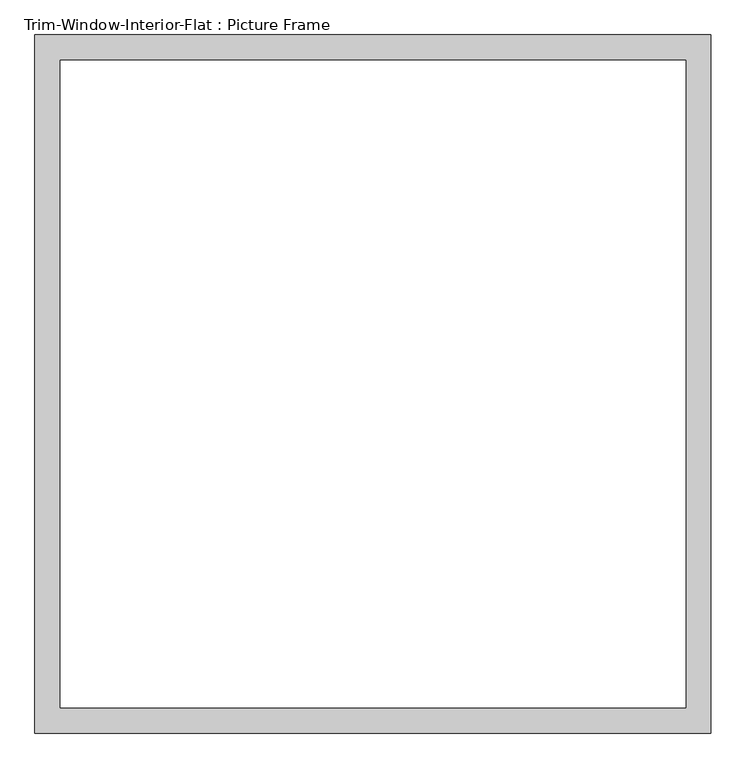
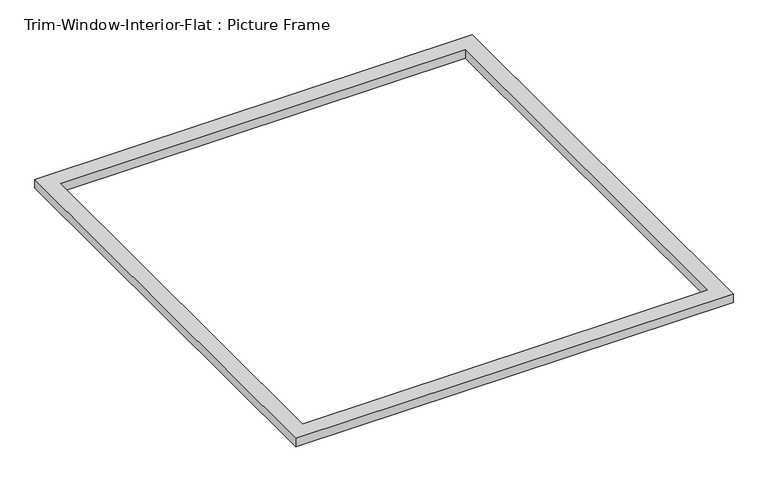
"""IFC4 building model written with IfcOpenShell, lengths in millimetres: proxy geometry, Trim-Window-Interior-Flat : Picture Frame."""

from ifc_helpers import new_model, si_unit, origin, origin_with_axes, place, context, project, spatial, polyline, outline, extrude, source, transform, mapped, element, save


def trim_window_interior_flat_picture_frame_c6096a02(model_context):
    return source(origin(), model_context, "Body", "SweptSolid", [
        extrude(outline(polyline([(768.35, 44.45), (768.35, -1543.05), (-768.35, -1543.05), (-768.35, 44.45), (768.35, 44.45)]), holes=[polyline([(711.2, -12.7), (-711.2, -12.7), (-711.2, -1485.9), (711.2, -1485.9), (711.2, -12.7)])]), origin_with_axes(), (0.0, 0.0, 1.0), 31.75),
    ])


if __name__ == "__main__":
    model = new_model("IFC4")
    model_context = context("Model", 3, world=origin())
    ifc_project = project(units=[si_unit("LENGTHUNIT", "METRE", prefix="MILLI")], contexts=[model_context])
    site = spatial("IfcSite", under=ifc_project)
    building = spatial("IfcBuilding", under=site)
    placement = place(None, origin())
    trim_window_interior_flat_picture_frame_shape = trim_window_interior_flat_picture_frame_c6096a02(model_context)
    element("IfcBuildingElementProxy", 1, Name="Trim-Window-Interior-Flat : Picture Frame", ObjectType="Trim-Window-Interior-Flat : Picture Frame", at=placement, inside=building, context=model_context, shape_type="MappedRepresentation", body=[
        mapped(trim_window_interior_flat_picture_frame_shape, transform((0.0, 0.0, 0.0), x_axis=(1.0, 0.0, 0.0), y_axis=(0.0, 1.0, 0.0), z_axis=(0.0, 0.0, 1.0))),
    ])
    save(model, "model.ifc")

# Revit data of these elements
# Type "Trim-Window-Interior-Flat : Picture Frame"
#   Trim Thickness_Picture Frame = 0' - 1 1/4"
#   Trim Width = 0' - 2 1/4"
#   Trim Thickness_with Sill = 0' - 0 3/4"
#   Sill Thickness = 0' - 1 1/4"
#   Opening Width [instance default] = 2' - 0"
#   Opening Height [instance default] = 3' - 0"
#   Default Elevation = 4' - 0"
#   Sill = no
#   Picture Frame = yes
#   Trim Material [instance default] = none
# Element 1 (IfcBuildingElementProxy, "Trim-Window-Interior-Flat : Picture Frame")
#   Opening Width = 4' - 9"
#   Opening Height = 4' - 11"
#   Trim Material = Wood - Stained
#   Materials on its faces: "Wood - Stained"
# Materials
#   "Wood - Stained": class "Wood", colour RGB 224 178 126, transparency 0, Cost = 0
